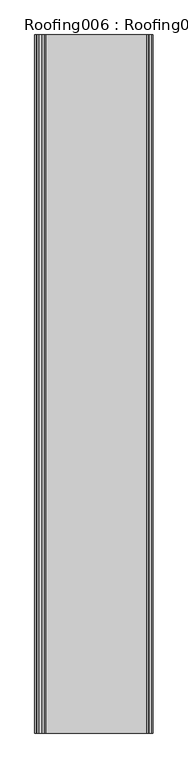
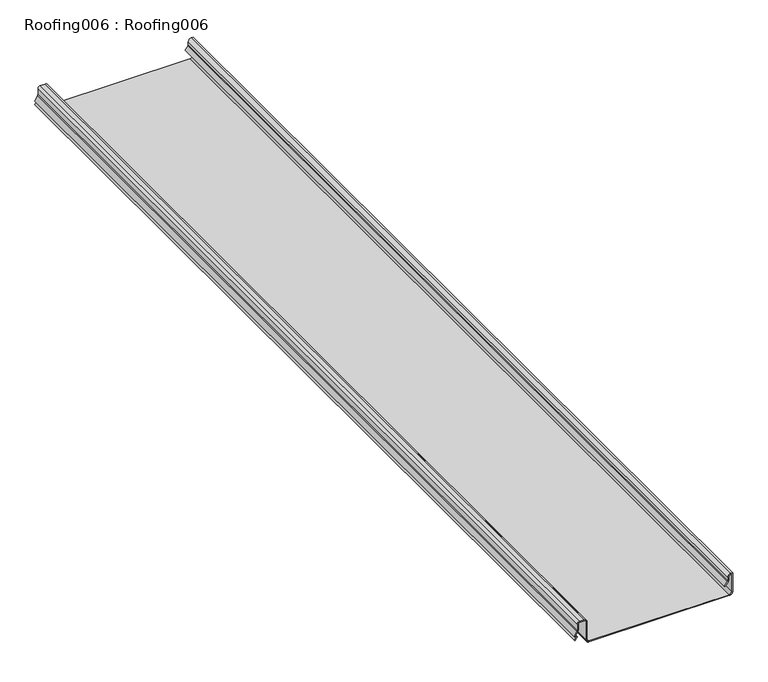
"""IFC4 building model written with IfcOpenShell, lengths in millimetres: proxy geometry, Roofing006 : Roofing006."""

import ifcopenshell
import ifcopenshell.guid

model = None  # the IFC model being written
_history = None  # IfcOwnerHistory: only IFC2X3 demands one
_inside = {}  # id of a spatial element -> (the spatial element, [elements in it])
_under = {}  # id of a project, library or spatial element -> (it, [spatial elements below it])
_declared = {}  # id of a project -> (the project, [libraries it declares])
_typed = {}  # id of a type object -> (the type object, [elements of that type])
_made_of = {}  # id of a material, layer set ... -> (it, [elements and type objects made of it])


def new_model(schema):
    """Start an empty IFC model of exactly this schema.

    Asked for "IFC4X3", IfcOpenShell would pick the latest addendum, in which some entities
    have other attributes; the version numbers below select the first issue.
    IFC2X3 requires an IfcOwnerHistory on every rooted entity: one is made here for all.
    """
    global model, _history
    if schema == "IFC4X3":
        model = ifcopenshell.file(schema_version=(4, 3, 0, 0))
    else:
        model = ifcopenshell.file(schema=schema)
    _inside.clear()
    _under.clear()
    _declared.clear()
    _typed.clear()
    _made_of.clear()
    _history = None
    if model.schema == "IFC2X3":
        org = make("IfcOrganization", Name="unknown")
        user = make(
            "IfcPersonAndOrganization",
            ThePerson=make("IfcPerson", FamilyName="unknown"),
            TheOrganization=org,
        )
        app = make(
            "IfcApplication",
            ApplicationDeveloper=org,
            Version="unknown",
            ApplicationFullName="unknown",
            ApplicationIdentifier="unknown",
        )
        _history = make(
            "IfcOwnerHistory",
            OwningUser=user,
            OwningApplication=app,
            ChangeAction="ADDED",
            CreationDate=0,
        )
    return model


def make(cls, **values):
    """One entity of the class cls with the attributes given. An attribute that is None is left unset."""
    return model.create_entity(
        cls, **{name: value for name, value in values.items() if value is not None}
    )


def rooted(cls, **values):
    """An entity with a GlobalId (a new one), such as an element, a storey or a relation."""
    return make(cls, GlobalId=ifcopenshell.guid.new(), OwnerHistory=_history, **values)


def si_unit(unit_type, name, prefix=None):
    """IfcSIUnit, for example si_unit("LENGTHUNIT", "METRE", prefix="MILLI")."""
    return make("IfcSIUnit", UnitType=unit_type, Prefix=prefix, Name=name)


def assignment(units):
    """IfcUnitAssignment: the units of a project."""
    return None if units is None else make("IfcUnitAssignment", Units=units)


def point(xyz):
    """IfcCartesianPoint."""
    return None if xyz is None else make("IfcCartesianPoint", Coordinates=xyz)


def direction(xyz):
    """IfcDirection."""
    return None if xyz is None else make("IfcDirection", DirectionRatios=xyz)


def frame(location, z_axis=None, x_axis=None):
    """IfcAxis2Placement3D, a coordinate frame: its origin and axes. An axis left out is left unset."""
    return make(
        "IfcAxis2Placement3D",
        Location=point(location),
        Axis=direction(z_axis),
        RefDirection=direction(x_axis),
    )


def frame_2d(location, x_axis=None):
    """IfcAxis2Placement2D, a coordinate frame in the plane: its origin and x axis."""
    return make(
        "IfcAxis2Placement2D", Location=point(location), RefDirection=direction(x_axis)
    )


def origin():
    """The frame at (0, 0, 0) with its axes left unset."""
    return frame((0.0, 0.0, 0.0))


def place(relative_to, where):
    """IfcLocalPlacement: puts the frame where relative to a parent placement (None: the world)."""
    return make(
        "IfcLocalPlacement", PlacementRelTo=relative_to, RelativePlacement=where
    )


def context(
    kind, dimensions, precision=None, world=None, true_north=None, identifier=None
):
    """IfcGeometricRepresentationContext, for example the 3D "Model" context."""
    return make(
        "IfcGeometricRepresentationContext",
        ContextIdentifier=identifier,
        ContextType=kind,
        CoordinateSpaceDimension=dimensions,
        Precision=precision,
        WorldCoordinateSystem=world,
        TrueNorth=true_north,
    )


def project(units=None, contexts=None):
    """IfcProject with its units and contexts."""
    return rooted(
        "IfcProject",
        Name="project",
        RepresentationContexts=contexts,
        UnitsInContext=assignment(units),
    )


def spatial(cls, under=None, at=None, **own):
    """A site, building, storey or space (cls), placed at a placement, below another one or the project."""
    s = rooted(cls, ObjectPlacement=at, **own)
    if under is not None:
        _under.setdefault(under.id(), (under, []))[1].append(s)
    return s


def polyline(points):
    """IfcPolyline through the points."""
    return make("IfcPolyline", Points=[point(p) for p in points])


def circle_curve(where, radius):
    """IfcCircle in the frame where."""
    return make("IfcCircle", Position=where, Radius=radius)


def trimmed(basis, trim1, trim2, sense, master):
    """IfcTrimmedCurve: the piece of a basis curve between two trims."""
    return make(
        "IfcTrimmedCurve",
        BasisCurve=basis,
        Trim1=trim1,
        Trim2=trim2,
        SenseAgreement=sense,
        MasterRepresentation=master,
    )


def segment(curve, same_sense, transition):
    """IfcCompositeCurveSegment."""
    return make(
        "IfcCompositeCurveSegment",
        Transition=transition,
        SameSense=same_sense,
        ParentCurve=curve,
    )


def composite_curve(segments, self_intersect=None):
    """IfcCompositeCurve: segments joined end to end."""
    return make("IfcCompositeCurve", Segments=segments, SelfIntersect=self_intersect)


def outline(outer, holes=None, kind="AREA"):
    """IfcArbitraryClosedProfileDef: a profile drawn as a closed curve; with holes, ...WithVoids."""
    if holes is None:
        return make("IfcArbitraryClosedProfileDef", ProfileType=kind, OuterCurve=outer)
    return make(
        "IfcArbitraryProfileDefWithVoids",
        ProfileType=kind,
        OuterCurve=outer,
        InnerCurves=holes,
    )


def extrude(swept, where, along, depth):
    """IfcExtrudedAreaSolid: the profile swept, set in the frame where, extruded along a direction by depth."""
    return make(
        "IfcExtrudedAreaSolid",
        SweptArea=swept,
        Position=where,
        ExtrudedDirection=direction(along),
        Depth=depth,
    )


def shape(context_of_items, identifier, shape_type, items):
    """IfcShapeRepresentation: the items that make up one representation, for example the "Body"."""
    return make(
        "IfcShapeRepresentation",
        ContextOfItems=context_of_items,
        RepresentationIdentifier=identifier,
        RepresentationType=shape_type,
        Items=items,
    )


def source(mapping_origin, context_of_items, identifier, shape_type, items):
    """IfcRepresentationMap: a shape defined once, which mapped items show again and again."""
    return make(
        "IfcRepresentationMap",
        MappingOrigin=mapping_origin,
        MappedRepresentation=shape(context_of_items, identifier, shape_type, items),
    )


def transform(
    local_origin,
    x_axis=None,
    y_axis=None,
    z_axis=None,
    scale=None,
    scale2=None,
    scale3=None,
    uniform=True,
):
    """IfcCartesianTransformationOperator3D, or its non-uniform kind. x_axis, y_axis, z_axis: its Axis1, 2, 3."""
    if uniform:
        return make(
            "IfcCartesianTransformationOperator3D",
            Axis1=direction(x_axis),
            Axis2=direction(y_axis),
            LocalOrigin=point(local_origin),
            Scale=scale,
            Axis3=direction(z_axis),
        )
    return make(
        "IfcCartesianTransformationOperator3DnonUniform",
        Axis1=direction(x_axis),
        Axis2=direction(y_axis),
        LocalOrigin=point(local_origin),
        Scale=scale,
        Axis3=direction(z_axis),
        Scale2=scale2,
        Scale3=scale3,
    )


def mapped(mapping_source, mapping_target):
    """IfcMappedItem: shows the shape of a source again, moved by a transform."""
    return make(
        "IfcMappedItem", MappingSource=mapping_source, MappingTarget=mapping_target
    )


def made_of(thing, what):
    """Note that an element or type object is made of a material, layer set ...; save() writes the relation."""
    if what is not None:
        _made_of.setdefault(what.id(), (what, []))[1].append(thing)
    return thing


def element(
    cls,
    number,
    at=None,
    inside=None,
    cuts=None,
    type_object=None,
    material=None,
    context=None,
    identifier="Body",
    shape_type=None,
    held_by="IfcProductDefinitionShape",
    body=None,
    shapes=None,
    **own,
):
    """One element of the class cls, such as IfcWall. Its Tag is "e" and its number.

    at: its placement. inside: the storey or other place that contains it. cuts: it is an
    opening in that element (IfcRelVoidsElement). A single representation is given by context,
    identifier, shape_type and body (its items); several are given by shapes. held_by: the class
    of the entity that holds the representations. save() writes the other relations.
    """
    e = rooted(cls, Tag="e%d" % number, ObjectPlacement=at, **own)
    if body is not None:
        shapes = [shape(context, identifier, shape_type, body)]
    if shapes is not None:
        e.Representation = make(held_by, Representations=shapes)
    if inside is not None:
        _inside.setdefault(inside.id(), (inside, []))[1].append(e)
    if cuts is not None:
        rooted(
            "IfcRelVoidsElement", RelatingBuildingElement=cuts, RelatedOpeningElement=e
        )
    if type_object is not None:
        _typed.setdefault(type_object.id(), (type_object, []))[1].append(e)
    return made_of(e, material)


def aggregate(whole, parts):
    """IfcRelAggregates: a whole, such as a stair, and the parts it consists of."""
    return rooted("IfcRelAggregates", RelatingObject=whole, RelatedObjects=parts)


def save(model, path):
    """Write the relations noted so far, then the file.

    IfcRelAggregates (storeys below a building ...), IfcRelContainedInSpatialStructure (elements
    in a storey), IfcRelDefinesByType, IfcRelAssociatesMaterial and IfcRelDeclares: one each for
    every whole, place, type object, material and project.
    """
    for whole, parts in _under.values():
        aggregate(whole, parts)
    for where, things in _inside.values():
        rooted(
            "IfcRelContainedInSpatialStructure",
            RelatedElements=things,
            RelatingStructure=where,
        )
    for kind, things in _typed.values():
        rooted("IfcRelDefinesByType", RelatedObjects=things, RelatingType=kind)
    for what, things in _made_of.values():
        rooted("IfcRelAssociatesMaterial", RelatedObjects=things, RelatingMaterial=what)
    for by, libraries in _declared.values():
        rooted("IfcRelDeclares", RelatingContext=by, RelatedDefinitions=libraries)
    model.write(path)


def roofing006_roofing006_02cdabe2(model_context):
    return source(origin(), model_context, "Body", "SweptSolid", [
        extrude(outline(composite_curve([segment(trimmed(circle_curve(frame_2d((42571.8416239, -1174.390951)), 5.08), [point((42568.8585944, -1170.279025))], [point((42571.8416239, -1169.310951))], False, "CARTESIAN"), True, "CONTINUOUS"), segment(polyline([(42571.8416239, -1169.310951), (42578.5981823, -1169.310951)]), True, "CONTINUOUS"), segment(trimmed(circle_curve(frame_2d((42578.5981823, -1164.230951)), 5.08), [point((42578.5981823, -1169.310951))], [point((42583.6781823, -1164.230951))], True, "CARTESIAN"), True, "CONTINUOUS"), segment(polyline([(42583.6781823, -1164.230951), (42583.6781823, -1162.6361463), (42543.9409948, -1162.6361463)]), True, "CONTINUOUS"), segment(trimmed(circle_curve(frame_2d((42543.9409948, -1167.7161463)), 5.08), [point((42543.9409948, -1162.6361463))], [point((42538.8609948, -1167.7161463))], True, "CARTESIAN"), True, "CONTINUOUS"), segment(polyline([(42538.8609948, -1167.7161463), (42538.8609948, -1467.9902283)]), True, "CONTINUOUS"), segment(trimmed(circle_curve(frame_2d((42543.9409948, -1467.9902283)), 5.08), [point((42538.8609948, -1467.9902283))], [point((42543.9409948, -1473.0702283))], True, "CARTESIAN"), True, "CONTINUOUS"), segment(polyline([(42543.9409948, -1473.0702283), (42585.5544323, -1473.0702283)]), True, "CONTINUOUS"), segment(trimmed(circle_curve(frame_2d((42585.5544323, -1478.1502283)), 5.08), [point((42585.5544323, -1473.0702283))], [point((42590.6344323, -1478.1502283))], False, "CARTESIAN"), True, "CONTINUOUS"), segment(polyline([(42590.6344323, -1478.1502283), (42590.6344323, -1488.1580052)]), True, "CONTINUOUS"), segment(trimmed(circle_curve(frame_2d((42585.5544323, -1488.1580052)), 5.08), [point((42590.6344323, -1488.1580052))], [point((42585.5544323, -1493.2380052))], False, "CARTESIAN"), True, "CONTINUOUS"), segment(polyline([(42585.5544323, -1493.2380052), (42572.3718581, -1493.2380052)]), True, "CONTINUOUS"), segment(trimmed(circle_curve(frame_2d((42572.3718581, -1498.3180052)), 5.08), [point((42572.3718581, -1493.2380052))], [point((42569.8678467, -1493.8980135))], True, "CARTESIAN"), True, "CONTINUOUS"), segment(polyline([(42569.8678467, -1493.8980135), (42559.3102135, -1499.8791185), (42556.8688073, -1495.715056), (42551.2672448, -1499.7140794), (42550.1051711, -1498.0863249), (42557.4874863, -1492.8160005), (42560.0388845, -1497.1676653), (42568.8820154, -1492.1578593)]), True, "CONTINUOUS"), segment(trimmed(circle_curve(frame_2d((42572.3718581, -1498.3180052)), 7.08), [point((42568.8820154, -1492.1578593))], [point((42572.3718581, -1491.2380052))], False, "CARTESIAN"), True, "CONTINUOUS"), segment(polyline([(42572.3718581, -1491.2380052), (42585.5544323, -1491.2380052)]), True, "CONTINUOUS"), segment(trimmed(circle_curve(frame_2d((42585.5544323, -1488.1580052)), 3.08), [point((42585.5544323, -1491.2380052))], [point((42588.6344323, -1488.1580052))], True, "CARTESIAN"), True, "CONTINUOUS"), segment(polyline([(42588.6344323, -1488.1580052), (42588.6344323, -1478.1502283)]), True, "CONTINUOUS"), segment(trimmed(circle_curve(frame_2d((42585.5544323, -1478.1502283)), 3.08), [point((42588.6344323, -1478.1502283))], [point((42585.5544323, -1475.0702283))], True, "CARTESIAN"), True, "CONTINUOUS"), segment(polyline([(42585.5544323, -1475.0702283), (42543.9409948, -1475.0702283)]), True, "CONTINUOUS"), segment(trimmed(circle_curve(frame_2d((42543.9409948, -1467.9902283)), 7.08), [point((42543.9409948, -1475.0702283))], [point((42536.8609948, -1467.9902283))], False, "CARTESIAN"), True, "CONTINUOUS"), segment(polyline([(42536.8609948, -1467.9902283), (42536.8609948, -1167.7161463)]), True, "CONTINUOUS"), segment(trimmed(circle_curve(frame_2d((42543.9409948, -1167.7161463)), 7.08), [point((42536.8609948, -1167.7161463))], [point((42543.9409948, -1160.6361463))], False, "CARTESIAN"), True, "CONTINUOUS"), segment(polyline([(42543.9409948, -1160.6361463), (42585.6781823, -1160.6361463), (42585.6781823, -1164.230951)]), True, "CONTINUOUS"), segment(trimmed(circle_curve(frame_2d((42578.5981823, -1164.230951)), 7.08), [point((42585.6781823, -1164.230951))], [point((42578.5981823, -1171.310951))], False, "CARTESIAN"), True, "CONTINUOUS"), segment(polyline([(42578.5981823, -1171.310951), (42571.8416239, -1171.310951)]), True, "CONTINUOUS"), segment(trimmed(circle_curve(frame_2d((42571.8416239, -1174.390951)), 3.08), [point((42571.8416239, -1171.310951))], [point((42570.0330155, -1171.8978935))], True, "CARTESIAN"), True, "CONTINUOUS"), segment(polyline([(42570.0330155, -1171.8978935), (42561.5588533, -1178.0455421), (42560.3844323, -1176.4266736), (42568.8585944, -1170.279025)]), True, "CONTINUOUS")], self_intersect=False)), frame((0.0, -1052.8906574, 0.0), z_axis=(0.0, 1.0, 0.0), x_axis=(0.0, 0.0, 1.0)), (0.0, 0.0, 1.0), 2000.0),
    ])


if __name__ == "__main__":
    model = new_model("IFC4")
    model_context = context("Model", 3, world=origin())
    ifc_project = project(units=[si_unit("LENGTHUNIT", "METRE", prefix="MILLI")], contexts=[model_context])
    site = spatial("IfcSite", under=ifc_project)
    building = spatial("IfcBuilding", under=site)
    placement = place(None, origin())
    roofing006_roofing006_shape = roofing006_roofing006_02cdabe2(model_context)
    element("IfcBuildingElementProxy", 1, Name="Roofing006 : Roofing006", ObjectType="Roofing006 : Roofing006", at=placement, inside=building, context=model_context, shape_type="MappedRepresentation", body=[
        mapped(roofing006_roofing006_shape, transform((0.0, 0.0, 0.0), x_axis=(1.0, 0.0, 0.0), y_axis=(0.0, 1.0, 0.0), z_axis=(0.0, 0.0, 1.0))),
    ])
    save(model, "model.ifc")

# Revit data of these elements
# Type "Roofing006 : Roofing006"
#   NameOverride = "Roofing006"
# Element 1 (IfcBuildingElementProxy, "Roofing006 : Roofing006")
#   Materials on its faces: "STANDING SEAM METAL ROOF"
# Materials
#   "STANDING SEAM METAL ROOF": class "Unassigned", colour RGB 128 128 128, transparency 0
